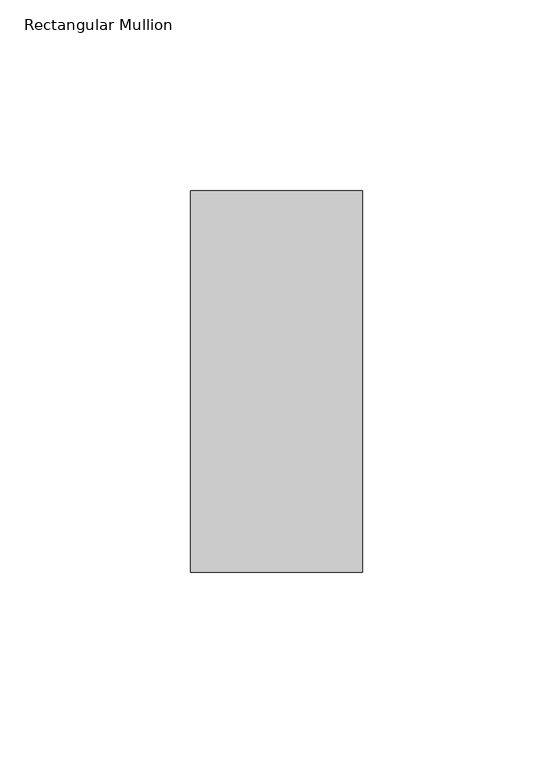
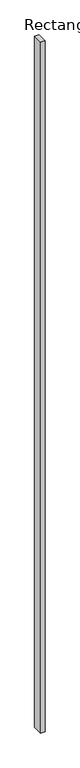
"""IFC4 building model written with IfcOpenShell, lengths in millimetres: member geometry, Rectangular Mullion : 알루미늄_Rectangular Cap_100 x 45."""

from ifc_helpers import new_model, si_unit, frame, origin, place, context, project, spatial, polyline, outline, extrude, source, transform, mapped, element, save


def rectangular_mullion_c7b7c2a1(model_context):
    return source(origin(), model_context, "Body", "SweptSolid", [
        extrude(outline(polyline([(0.0, 50.0), (0.0, -50.0), (-45.0, -50.0), (-45.0, 50.0), (0.0, 50.0)])), frame((0.0, 0.0, -7160.0000001), z_axis=(0.0, 0.0, 1.0), x_axis=(1.0, 0.0, 0.0)), (0.0, 0.0, 1.0), 7160.0000001),
    ])


if __name__ == "__main__":
    model = new_model("IFC4")
    model_context = context("Model", 3, world=origin())
    ifc_project = project(units=[si_unit("LENGTHUNIT", "METRE", prefix="MILLI")], contexts=[model_context])
    site = spatial("IfcSite", under=ifc_project)
    building = spatial("IfcBuilding", under=site)
    placement = place(None, origin())
    rectangular_mullion_shape = rectangular_mullion_c7b7c2a1(model_context)
    element("IfcMember", 1, ObjectType="Rectangular Mullion : 알루미늄_Rectangular Cap_100 x 45", at=placement, inside=building, context=model_context, shape_type="MappedRepresentation", body=[
        mapped(rectangular_mullion_shape, transform((0.0, 0.0, 0.0), x_axis=(1.0, 0.0, 0.0), y_axis=(0.0, 1.0, 0.0), z_axis=(0.0, 0.0, 1.0))),
    ])
    save(model, "model.ifc")

# Revit data of these elements
# Type "Rectangular Mullion : 알루미늄_Rectangular Cap_100 x 45"
#   built-in parameter 1007304 = 0.328084 (stored number, unit not read)
#   built-in parameter 1007301 = 0.0738189 (stored number, unit not read)
#   built-in parameter 1007300 = 0.0738189 (stored number, unit not read)
# Element 1 (IfcMember, "Rectangular Mullion : 알루미늄_Rectangular Cap_100 x 45")
#   Materials on its faces: "00_Metal_Stainless Steel"
# Materials
#   "00_Metal_Stainless Steel": class "Metal", colour RGB 148 148 148, transparency 0, Description = "Steel", Cost = 0
